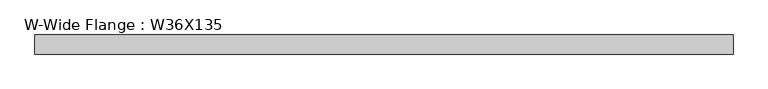
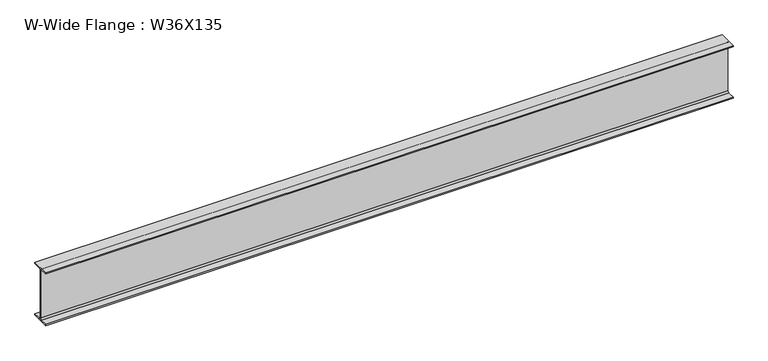
"""IFC4 building model written with IfcOpenShell, lengths in millimetres: beam geometry, W-Wide Flange : W36X135."""

from ifc_helpers import new_model, si_unit, point, frame, frame_2d, origin, place, context, project, spatial, polyline, circle_curve, trimmed, segment, composite_curve, outline, extrude, source, transform, mapped, element, save


def w_wide_flange_w36x135_1d218eeb(model_context):
    return source(origin(), model_context, "Body", "SweptSolid", [
        extrude(outline(composite_curve([segment(polyline([(152.4, -432.054), (152.4, -452.12), (-152.4, -452.12), (-152.4, -432.054), (-30.4165, -432.054)]), True, "CONTINUOUS"), segment(trimmed(circle_curve(frame_2d((-30.4165, -409.2575)), 22.7965), [point((-30.4165, -432.054))], [point((-7.62, -409.2575))], True, "CARTESIAN"), True, "CONTINUOUS"), segment(polyline([(-7.62, -409.2575), (-7.62, 409.2575)]), True, "CONTINUOUS"), segment(trimmed(circle_curve(frame_2d((-30.4165, 409.2575)), 22.7965), [point((-7.62, 409.2575))], [point((-30.4165, 432.054))], True, "CARTESIAN"), True, "CONTINUOUS"), segment(polyline([(-30.4165, 432.054), (-152.4, 432.054), (-152.4, 452.12), (152.4, 452.12), (152.4, 432.054), (30.4165, 432.054)]), True, "CONTINUOUS"), segment(trimmed(circle_curve(frame_2d((30.4165, 409.2575)), 22.7965), [point((30.4165, 432.054))], [point((7.62, 409.2575))], True, "CARTESIAN"), True, "CONTINUOUS"), segment(polyline([(7.62, 409.2575), (7.62, -409.2575)]), True, "CONTINUOUS"), segment(trimmed(circle_curve(frame_2d((30.4165, -409.2575)), 22.7965), [point((7.62, -409.2575))], [point((30.4165, -432.054))], True, "CARTESIAN"), True, "CONTINUOUS"), segment(polyline([(30.4165, -432.054), (152.4, -432.054)]), True, "CONTINUOUS")], self_intersect=False)), frame((-5634.0457682, 0.0, 0.0), z_axis=(1.0, 0.0, 0.0), x_axis=(0.0, 1.0, 0.0)), (0.0, 0.0, 1.0), 11134.3653879),
    ])


if __name__ == "__main__":
    model = new_model("IFC4")
    model_context = context("Model", 3, world=origin())
    ifc_project = project(units=[si_unit("LENGTHUNIT", "METRE", prefix="MILLI")], contexts=[model_context])
    site = spatial("IfcSite", under=ifc_project)
    building = spatial("IfcBuilding", under=site)
    placement = place(None, origin())
    w_wide_flange_w36x135_shape = w_wide_flange_w36x135_1d218eeb(model_context)
    element("IfcBeam", 1, ObjectType="W-Wide Flange : W36X135", at=placement, inside=building, context=model_context, shape_type="MappedRepresentation", body=[
        mapped(w_wide_flange_w36x135_shape, transform((0.0, 0.0, 0.0), x_axis=(1.0, 0.0, 0.0), y_axis=(0.0, 1.0, 0.0), z_axis=(0.0, 0.0, 1.0))),
    ])
    save(model, "model.ifc")

# Revit data of these elements
# Type "W-Wide Flange : W36X135"
#   Assembly Code = "B10"
#   W = 135
#   Length [instance default] = 1524 mm
#   bf = 304.8 mm
#   d = 904.24 mm
#   k = 42.863 mm
#   k2 = 22.797 mm
#   tf = 20.066 mm
#   tw = 15.24 mm
#   A = 0.0256129 m²
#   Structural Material [instance default] = Steel ASTM A992
# Element 1 (IfcBeam, "W-Wide Flange : W36X135")
#   Structural Material = Aluminum, Anodized Red
#   Materials on its faces: "Aluminum, Anodized Red"
# Materials
#   "Steel ASTM A992": class "Metal", colour RGB 128 0 0, transparency 0, Description = "Structural steel 50ksi", Cost = 0
#   "Aluminum, Anodized Red": class "Metal", colour RGB 120 120 120, transparency 0, Description = "Anodized aluminum, red", Cost = 0
